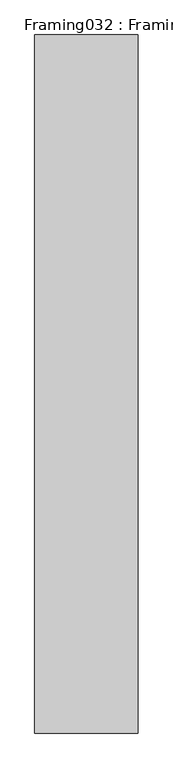
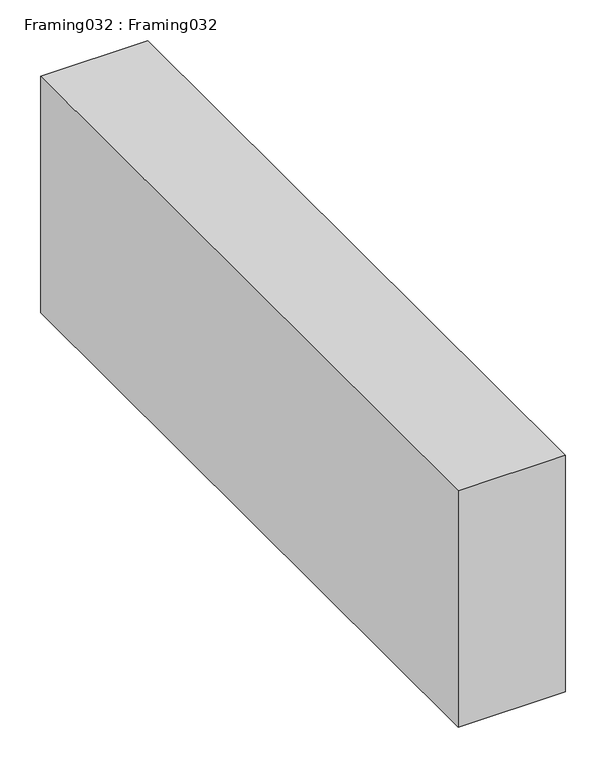
"""IFC4 building model written with IfcOpenShell, lengths in millimetres: proxy geometry, Framing032 : Framing032."""

from ifc_helpers import new_model, si_unit, frame, origin, place, context, project, spatial, polyline, outline, extrude, source, transform, mapped, element, save


def framing032_framing032_c2b2e796(model_context):
    return source(origin(), model_context, "Body", "SweptSolid", [
        extrude(outline(polyline([(13687.8178845, -4374.0175368), (13687.8178845, -5402.7175368), (13535.4178845, -5402.7175368), (13535.4178845, -4374.0175368), (13687.8178845, -4374.0175368)])), frame((0.0, 0.0, 39757.096), z_axis=(0.0, 0.0, 1.0), x_axis=(1.0, 0.0, 0.0)), (0.0, 0.0, 1.0), 355.6),
    ])


if __name__ == "__main__":
    model = new_model("IFC4")
    model_context = context("Model", 3, world=origin())
    ifc_project = project(units=[si_unit("LENGTHUNIT", "METRE", prefix="MILLI")], contexts=[model_context])
    site = spatial("IfcSite", under=ifc_project)
    building = spatial("IfcBuilding", under=site)
    placement = place(None, origin())
    framing032_framing032_shape = framing032_framing032_c2b2e796(model_context)
    element("IfcBuildingElementProxy", 1, Name="Framing032 : Framing032", ObjectType="Framing032 : Framing032", at=placement, inside=building, context=model_context, shape_type="MappedRepresentation", body=[
        mapped(framing032_framing032_shape, transform((0.0, 0.0, 0.0), x_axis=(1.0, 0.0, 0.0), y_axis=(0.0, 1.0, 0.0), z_axis=(0.0, 0.0, 1.0))),
    ])
    save(model, "model.ifc")

# Revit data of these elements
# Type "Framing032 : Framing032"
#   NameOverride = "Framing032"
# Element 1 (IfcBuildingElementProxy, "Framing032 : Framing032")
#   Materials on its faces: "WOOD FRAMING (SEE STRUCT DWGS)"
# Materials
#   "WOOD FRAMING (SEE STRUCT DWGS)": class "Unassigned", colour RGB 224 188 168, transparency 0, Cost = 0
